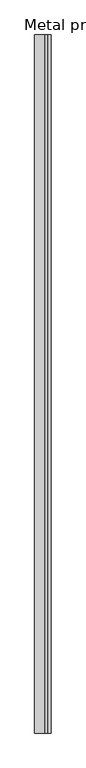
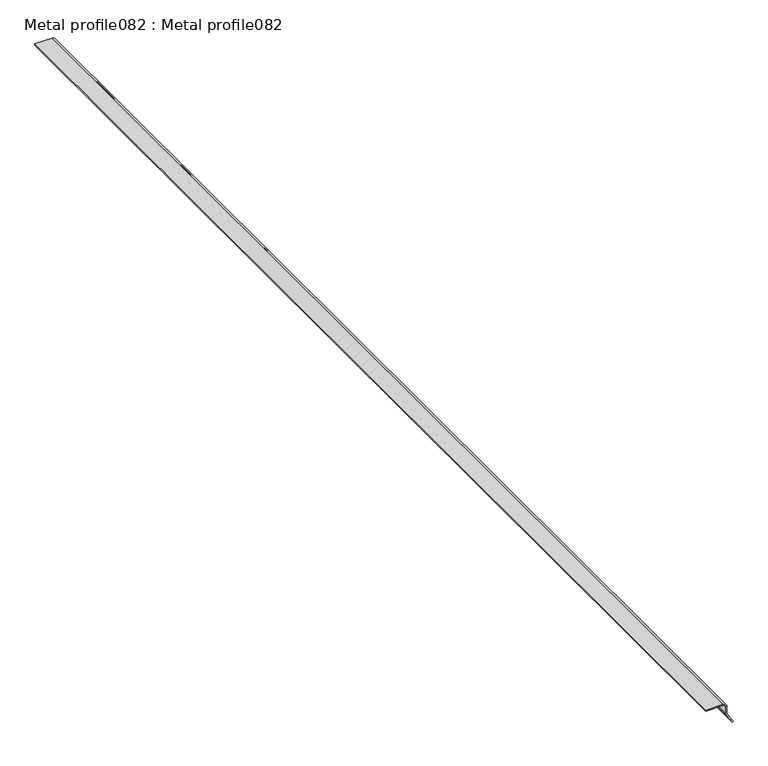
"""IFC4 building model written with IfcOpenShell, lengths in millimetres: proxy geometry, Metal profile082 : Metal profile082."""

from ifc_helpers import new_model, si_unit, point, frame, frame_2d, origin, place, context, project, spatial, polyline, circle_curve, trimmed, segment, composite_curve, outline, extrude, source, transform, mapped, element, save


def metal_profile082_metal_profile082_57c9ab2e(model_context):
    return source(origin(), model_context, "Body", "SweptSolid", [
        extrude(outline(composite_curve([segment(polyline([(40166.609375, -7147.3191654), (40166.609375, -7117.5724857)]), True, "CONTINUOUS"), segment(trimmed(circle_curve(frame_2d((40162.259375, -7117.5724857)), 4.35), [point((40166.609375, -7117.5724857))], [point((40162.259375, -7113.2224857))], True, "CARTESIAN"), True, "CONTINUOUS"), segment(polyline([(40162.259375, -7113.2224857), (40151.208717, -7113.2224857)]), True, "CONTINUOUS"), segment(trimmed(circle_curve(frame_2d((40151.208717, -7104.8724857)), 8.35), [point((40151.208717, -7113.2224857))], [point((40146.8542568, -7111.9971735))], False, "CARTESIAN"), True, "CONTINUOUS"), segment(polyline([(40146.8542568, -7111.9971735), (40130.8202968, -7102.1975524), (40131.8632813, -7100.4910404), (40147.8972413, -7110.2906615)]), True, "CONTINUOUS"), segment(trimmed(circle_curve(frame_2d((40151.208717, -7104.8724857)), 6.35), [point((40147.8972413, -7110.2906615))], [point((40151.208717, -7111.2224857))], True, "CARTESIAN"), True, "CONTINUOUS"), segment(polyline([(40151.208717, -7111.2224857), (40162.259375, -7111.2224857)]), True, "CONTINUOUS"), segment(trimmed(circle_curve(frame_2d((40162.259375, -7117.5724857)), 6.35), [point((40162.259375, -7111.2224857))], [point((40168.609375, -7117.5724857))], False, "CARTESIAN"), True, "CONTINUOUS"), segment(polyline([(40168.609375, -7117.5724857), (40168.609375, -7147.3191654), (40166.609375, -7147.3191654)]), True, "CONTINUOUS")], self_intersect=False)), frame((0.0, 7982.1531721, 0.0), z_axis=(0.0, 1.0, 0.0), x_axis=(0.0, 0.0, 1.0)), (0.0, 0.0, 1.0), 2000.0),
    ])


if __name__ == "__main__":
    model = new_model("IFC4")
    model_context = context("Model", 3, world=origin())
    ifc_project = project(units=[si_unit("LENGTHUNIT", "METRE", prefix="MILLI")], contexts=[model_context])
    site = spatial("IfcSite", under=ifc_project)
    building = spatial("IfcBuilding", under=site)
    placement = place(None, origin())
    metal_profile082_metal_profile082_shape = metal_profile082_metal_profile082_57c9ab2e(model_context)
    element("IfcBuildingElementProxy", 1, Name="Metal profile082 : Metal profile082", ObjectType="Metal profile082 : Metal profile082", at=placement, inside=building, context=model_context, shape_type="MappedRepresentation", body=[
        mapped(metal_profile082_metal_profile082_shape, transform((0.0, 0.0, 0.0), x_axis=(1.0, 0.0, 0.0), y_axis=(0.0, 1.0, 0.0), z_axis=(0.0, 0.0, 1.0))),
    ])
    save(model, "model.ifc")

# Revit data of these elements
# Type "Metal profile082 : Metal profile082"
#   NameOverride = "Metal profile082"
# Element 1 (IfcBuildingElementProxy, "Metal profile082 : Metal profile082")
#   Materials on its faces: "ANGLE TRIM"
# Materials
#   "ANGLE TRIM": class "Unassigned", colour RGB 250 255 0, transparency 0
